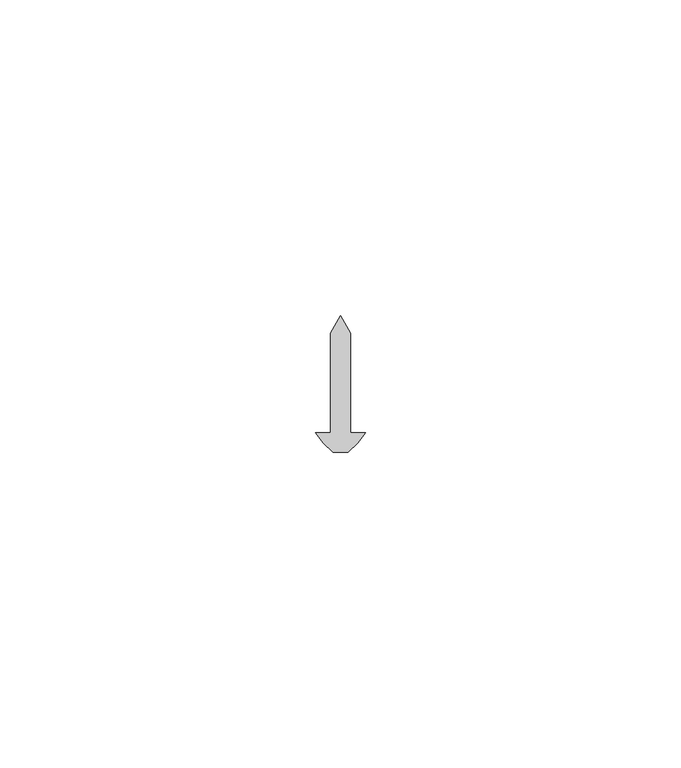
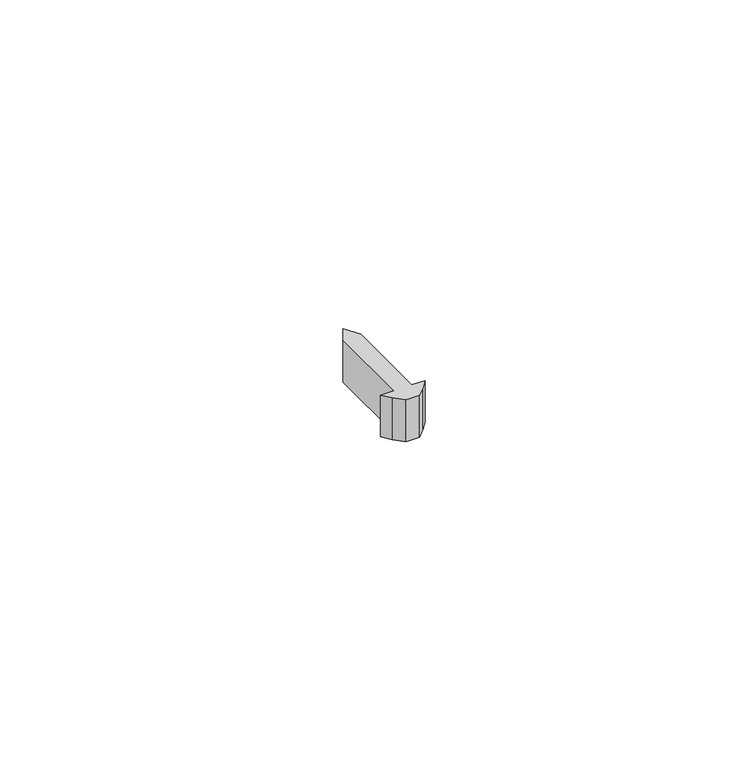
"""IFC4 building model written with IfcOpenShell, lengths in millimetres: proxy geometry, Generic Models 7:Generic Models 1:3:Generic Models 1:3 : Generic Models 7:Generic Models 1:305549:3:Generic Models 1:3:Generic Models 1:3 : Generic Models 7:Generic Models 1:305549:3 : Generic Models 7:Generic Models 1:3:Generic Models 1:3 : Generic Models 7:Generic Models 1:305549:301244:40 : Generic Models 7:Generic Models 1:3:Generic Models 1:3 : Generic Models 7:Generic Models 1:305549:3:Generic Models 1:3:Generic Models 1:3 : Generic Models 7:Generic Models 1:305549:3 : Generic Models 7:Generic Models 1:3:Generic Models 1:3 : Generic Models 7:Generic Models 1:305549:301244:308848."""

from ifc_helpers import new_model, si_unit, frame, origin, place, context, project, spatial, polyline, outline, extrude, source, transform, mapped, element, save


def generic_models_2754226f(model_context):
    return source(origin(), model_context, "Body", "SweptSolid", [
        extrude(outline(polyline([(593771.4242239, -579084.8288841), (593773.8054739, -579084.8288841), (593772.5872784, -579086.3559421), (593771.0353882, -579087.9078323), (593768.6380597, -579087.9078323), (593767.0861695, -579086.3559421), (593765.8679739, -579084.8288841), (593768.2492239, -579084.8288841), (593768.2492239, -579069.0196286), (593769.8367239, -579066.2699979), (593771.4242239, -579069.0196286), (593771.4242239, -579084.8288841)])), frame((0.0, 0.0, 1237.45625), z_axis=(0.0, 0.0, 1.0), x_axis=(1.0, 0.0, 0.0)), (0.0, 0.0, 1.0), 7.9375),
    ])


if __name__ == "__main__":
    model = new_model("IFC4")
    model_context = context("Model", 3, world=origin())
    ifc_project = project(units=[si_unit("LENGTHUNIT", "METRE", prefix="MILLI")], contexts=[model_context])
    site = spatial("IfcSite", under=ifc_project)
    building = spatial("IfcBuilding", under=site)
    placement = place(None, origin())
    generic_models_shape = generic_models_2754226f(model_context)
    element("IfcBuildingElementProxy", 1, Name="Generic Models 7:Generic Models 1:3:Generic Models 1:3 : Generic Models 7:Generic Models 1:305549:3:Generic Models 1:3:Generic Models 1:3 : Generic Models 7:Generic Models 1:305549:3 : Generic Models 7:Generic Models 1:3:Generic Models 1:3 : Generic Models 7:Generic Models 1:305549:301244:40 : Generic Models 7:Generic Models 1:3:Generic Models 1:3 : Generic Models 7:Generic Models 1:305549:3:Generic Models 1:3:Generic Models 1:3 : Generic Models 7:Generic Models 1:305549:3 : Generic Models 7:Generic Models 1:3:Generic Models 1:3 : Generic Models 7:Generic Models 1:305549:301244:308848", ObjectType="Generic Models 7:Generic Models 1:3:Generic Models 1:3 : Generic Models 7:Generic Models 1:305549:3:Generic Models 1:3:Generic Models 1:3 : Generic Models 7:Generic Models 1:305549:3 : Generic Models 7:Generic Models 1:3:Generic Models 1:3 : Generic Models 7:Generic Models 1:305549:301244:40 : Generic Models 7:Generic Models 1:3:Generic Models 1:3 : Generic Models 7:Generic Models 1:305549:3:Generic Models 1:3:Generic Models 1:3 : Generic Models 7:Generic Models 1:305549:3 : Generic Models 7:Generic Models 1:3:Generic Models 1:3 : Generic Models 7:Generic Models 1:305549:301244:308848", at=placement, inside=building, context=model_context, shape_type="MappedRepresentation", body=[
        mapped(generic_models_shape, transform((0.0, 0.0, 0.0), x_axis=(1.0, 0.0, 0.0), y_axis=(0.0, 1.0, 0.0), z_axis=(0.0, 0.0, 1.0))),
    ])
    save(model, "model.ifc")

# Revit data of these elements
# Type "Generic Models 7:Generic Models 1:3:Generic Models 1:3 : Generic Models 7:Generic Models 1:305549:3:Generic Models 1:3:Generic Models 1:3 : Generic Models 7:Generic Models 1:305549:3 : Generic Models 7:Generic Models 1:3:Generic Models 1:3 : Generic Models 7:Generic Models 1:305549:301244:40 : Generic Models 7:Generic Models 1:3:Generic Models 1:3 : Generic Models 7:Generic Models 1:305549:3:Generic Models 1:3:Generic Models 1:3 : Generic Models 7:Generic Models 1:305549:3 : Generic Models 7:Generic Models 1:3:Generic Models 1:3 : Generic Models 7:Generic Models 1:305549:301244:308848"
#   NameOverride = "Generic Models 7:Generic Models 1:3:Generic Models 1:3 : Generic Models 7:Generic Models 1:305549:3:Generic Models 1:3:Generic Models 1:3 : Generic Models 7:Generic Models 1:305549:3 : Generic Models 7:Generic Models 1:3:Generic Models 1:3 : Generic Models 7:Generic Models 1:305549:301244:308848"
#   ObjectTypeOverride = "Generic Models 1:3:Generic Models 1:3 : Generic Models 7:Generic Models 1:305549:3 : Generic Models 7:Generic Models 1:3:Generic Models 1:3 : Generic Models 7:Generic Models 1:305549:301244"
#   Reference = "Generic Models 1"
#   Tag = "308848"
# Element 1 (IfcBuildingElementProxy, "Generic Models 7:Generic Models 1:3:Generic Models 1:3 : Generic Models 7:Generic Models 1:305549:3:Generic Models 1:3:Generic Models 1:3 : Generic Models 7:Generic Models 1:305549:3 : Generic Models 7:Generic Models 1:3:Generic Models 1:3 : Generic Models 7:Generic Models 1:305549:301244:40 : Generic Models 7:Generic Models 1:3:Generic Models 1:3 : Generic Models 7:Generic Models 1:305549:3:Generic Models 1:3:Generic Models 1:3 : Generic Models 7:Generic Models 1:305549:3 : Generic Models 7:Generic Models 1:3:Generic Models 1:3 : Generic Models 7:Generic Models 1:305549:301244:308848")
#   Materials on its faces: "FASTENERS (T.B.D)"
# Materials
#   "FASTENERS (T.B.D)": class "Generic", colour RGB 120 120 120, transparency 0, Cost = 0
